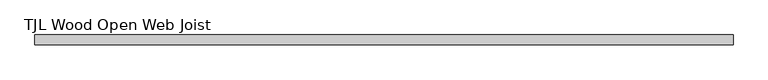
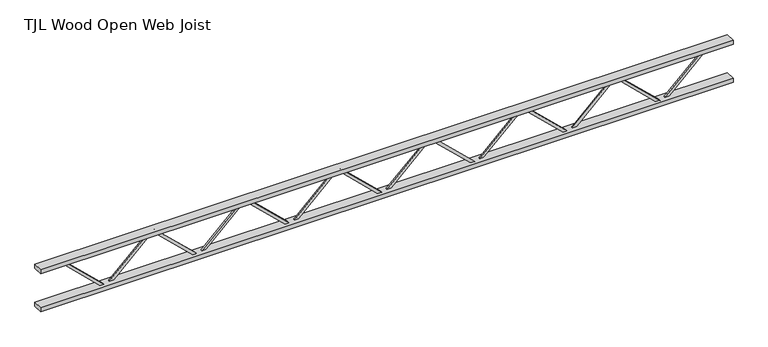
"""IFC4 building model written with IfcOpenShell, lengths in millimetres: beam geometry, TJL Wood Open Web Joist."""

from ifc_helpers import new_model, si_unit, frame, origin, place, context, project, spatial, polyline, outline, extrude, source, transform, mapped, element, save


def tjl_wood_open_web_joist_c41eeaf0(model_context):
    return source(origin(), model_context, "Body", "SweptSolid", [
        extrude(outline(polyline([(171.45, 2122.1473214), (196.85, 2122.1473214), (196.85, 2104.3636517), (-171.45, 1718.0341875), (-171.45, 1672.3178571), (-196.85, 1672.3178571), (-196.85, 1728.2015268), (171.45, 2114.5309911), (171.45, 2122.1473214)])), frame((0.0, 0.0, 0.0), z_axis=(0.0, 1.0, 0.0), x_axis=(0.0, 0.0, 1.0)), (0.0, 0.0, 1.0), 12.7),
        extrude(outline(polyline([(196.85, 1273.2883929), (171.45, 1273.2883929), (171.45, 1280.9047232), (-196.85, 1667.2341875), (-196.85, 1723.1178571), (-171.45, 1723.1178571), (-171.45, 1677.4015268), (196.85, 1291.0720625), (196.85, 1273.2883929)])), frame((0.0, -12.7, 0.0), z_axis=(0.0, 1.0, 0.0), x_axis=(0.0, 0.0, 1.0)), (0.0, 0.0, 1.0), 12.7),
        extrude(outline(polyline([(171.45, 1273.2883929), (196.85, 1273.2883929), (196.85, 1255.5047232), (-171.45, 869.1752589), (-171.45, 823.4589286), (-196.85, 823.4589286), (-196.85, 879.3425983), (171.45, 1265.6720625), (171.45, 1273.2883929)])), frame((0.0, 0.0, 0.0), z_axis=(0.0, 1.0, 0.0), x_axis=(0.0, 0.0, 1.0)), (0.0, 0.0, 1.0), 12.7),
        extrude(outline(polyline([(196.85, 424.4294643), (171.45, 424.4294643), (171.45, 432.0457946), (-196.85, 818.3752589), (-196.85, 874.2589286), (-171.45, 874.2589286), (-171.45, 828.5425983), (196.85, 442.213134), (196.85, 424.4294643)])), frame((0.0, -12.7, 0.0), z_axis=(0.0, 1.0, 0.0), x_axis=(0.0, 0.0, 1.0)), (0.0, 0.0, 1.0), 12.7),
        extrude(outline(polyline([(171.45, 424.4294643), (196.85, 424.4294643), (196.85, 406.6457946), (-171.45, 20.3163303), (-171.45, -25.4), (-196.85, -25.4), (-196.85, 30.4836697), (171.45, 416.813134), (171.45, 424.4294643)])), frame((0.0, 0.0, 0.0), z_axis=(0.0, 1.0, 0.0), x_axis=(0.0, 0.0, 1.0)), (0.0, 0.0, 1.0), 12.7),
        extrude(outline(polyline([(196.85, -424.4294643), (171.45, -424.4294643), (171.45, -416.813134), (-196.85, -30.4836697), (-196.85, 25.4), (-171.45, 25.4), (-171.45, -20.3163303), (196.85, -406.6457946), (196.85, -424.4294643)])), frame((0.0, -12.7, 0.0), z_axis=(0.0, 1.0, 0.0), x_axis=(0.0, 0.0, 1.0)), (0.0, 0.0, 1.0), 12.7),
        extrude(outline(polyline([(171.45, -424.4294643), (196.85, -424.4294643), (196.85, -442.213134), (-171.45, -828.5425983), (-171.45, -874.2589286), (-196.85, -874.2589286), (-196.85, -818.3752589), (171.45, -432.0457946), (171.45, -424.4294643)])), frame((0.0, 0.0, 0.0), z_axis=(0.0, 1.0, 0.0), x_axis=(0.0, 0.0, 1.0)), (0.0, 0.0, 1.0), 12.7),
        extrude(outline(polyline([(196.85, -1273.2883929), (171.45, -1273.2883929), (171.45, -1265.6720625), (-196.85, -879.3425983), (-196.85, -823.4589286), (-171.45, -823.4589286), (-171.45, -869.1752589), (196.85, -1255.5047232), (196.85, -1273.2883929)])), frame((0.0, -12.7, 0.0), z_axis=(0.0, 1.0, 0.0), x_axis=(0.0, 0.0, 1.0)), (0.0, 0.0, 1.0), 12.7),
        extrude(outline(polyline([(171.45, -1273.2883929), (196.85, -1273.2883929), (196.85, -1291.0720625), (-171.45, -1677.4015268), (-171.45, -1723.1178571), (-196.85, -1723.1178571), (-196.85, -1667.2341875), (171.45, -1280.9047232), (171.45, -1273.2883929)])), frame((0.0, 0.0, 0.0), z_axis=(0.0, 1.0, 0.0), x_axis=(0.0, 0.0, 1.0)), (0.0, 0.0, 1.0), 12.7),
        extrude(outline(polyline([(196.85, -2122.1473214), (171.45, -2122.1473214), (171.45, -2114.5309911), (-196.85, -1728.2015268), (-196.85, -1672.3178571), (-171.45, -1672.3178571), (-171.45, -1718.0341875), (196.85, -2104.3636517), (196.85, -2122.1473214)])), frame((0.0, -12.7, 0.0), z_axis=(0.0, 1.0, 0.0), x_axis=(0.0, 0.0, 1.0)), (0.0, 0.0, 1.0), 12.7),
        extrude(outline(polyline([(171.45, 2971.00625), (196.85, 2971.00625), (196.85, 2953.2225803), (-171.45, 2566.893116), (-171.45, 2521.1767857), (-196.85, 2521.1767857), (-196.85, 2577.0604554), (171.45, 2963.3899197), (171.45, 2971.00625)])), frame((0.0, 0.0, 0.0), z_axis=(0.0, 1.0, 0.0), x_axis=(0.0, 0.0, 1.0)), (0.0, 0.0, 1.0), 12.7),
        extrude(outline(polyline([(196.85, 2122.1473214), (171.45, 2122.1473214), (171.45, 2129.7636517), (-196.85, 2516.093116), (-196.85, 2571.9767857), (-171.45, 2571.9767857), (-171.45, 2526.2604554), (196.85, 2139.9309911), (196.85, 2122.1473214)])), frame((0.0, -12.7, 0.0), z_axis=(0.0, 1.0, 0.0), x_axis=(0.0, 0.0, 1.0)), (0.0, 0.0, 1.0), 12.7),
        extrude(outline(polyline([(171.45, -2122.1473214), (196.85, -2122.1473214), (196.85, -2139.9309911), (-171.45, -2526.2604554), (-171.45, -2571.9767857), (-196.85, -2571.9767857), (-196.85, -2516.093116), (171.45, -2129.7636517), (171.45, -2122.1473214)])), frame((0.0, 0.0, 0.0), z_axis=(0.0, 1.0, 0.0), x_axis=(0.0, 0.0, 1.0)), (0.0, 0.0, 1.0), 12.7),
        extrude(outline(polyline([(196.85, -2971.00625), (171.45, -2971.00625), (171.45, -2963.3899197), (-196.85, -2577.0604554), (-196.85, -2521.1767857), (-171.45, -2521.1767857), (-171.45, -2566.893116), (196.85, -2953.2225803), (196.85, -2971.00625)])), frame((0.0, -12.7, 0.0), z_axis=(0.0, 1.0, 0.0), x_axis=(0.0, 0.0, 1.0)), (0.0, 0.0, 1.0), 12.7),
        extrude(outline(polyline([(3174.20625, 44.45), (3174.20625, -44.45), (-3174.20625, -44.45), (-3174.20625, 44.45), (3174.20625, 44.45)])), frame((0.0, 0.0, 165.1), z_axis=(0.0, 0.0, 1.0), x_axis=(1.0, 0.0, 0.0)), (0.0, 0.0, 1.0), 38.1),
        extrude(outline(polyline([(3174.20625, 44.45), (3174.20625, -44.45), (-3174.20625, -44.45), (-3174.20625, 44.45), (3174.20625, 44.45)])), frame((0.0, 0.0, -203.2), z_axis=(0.0, 0.0, 1.0), x_axis=(1.0, 0.0, 0.0)), (0.0, 0.0, 1.0), 38.1),
    ])


if __name__ == "__main__":
    model = new_model("IFC4")
    model_context = context("Model", 3, world=origin())
    ifc_project = project(units=[si_unit("LENGTHUNIT", "METRE", prefix="MILLI")], contexts=[model_context])
    site = spatial("IfcSite", under=ifc_project)
    building = spatial("IfcBuilding", under=site)
    placement = place(None, origin())
    tjl_wood_open_web_joist_shape = tjl_wood_open_web_joist_c41eeaf0(model_context)
    element("IfcBeam", 1, ObjectType="TJL Wood Open Web Joist : 16\" PREENGINEERED FLOOR TRUSS", at=placement, inside=building, context=model_context, shape_type="MappedRepresentation", body=[
        mapped(tjl_wood_open_web_joist_shape, transform((0.0, 0.0, 0.0), x_axis=(1.0, 0.0, 0.0), y_axis=(0.0, 1.0, 0.0), z_axis=(0.0, 0.0, 1.0))),
    ])
    save(model, "model.ifc")

# Revit data of these elements
# Type "TJL Wood Open Web Joist : 16\" PREENGINEERED FLOOR TRUSS"
#   Web Thickness = 0' - 1"
#   Web Leg = 0' - 1"
#   Start Offset [instance default] = 0' - 0"
#   Top Chord Start Extension [instance default] = 0' - 0"
#   PanelArrayLength [instance default] = 22' - 8"
#   Depth = 1' - 4"
#   PanelWidth [instance default] = 2' - 6.22222"
#   Offset Length 2 [instance default] = 0' - 8"
#   Offset Length 1 [instance default] = 0' - 8"
#   End Panel [instance default] = 0' - 8"
#   End Offset [instance default] = 0' - 0"
#   Top Chord End Extension [instance default] = 0' - 0"
#   Chord Width = 0' - 3 1/2"
#   Chord Depth = 0' - 1 1/2"
#   Bottom Chord Start Extension [instance default] = 0' - 0"
#   Bottom Chord End Extension [instance default] = 0' - 0"
#   Length [instance default] = 24' - 0"
#   PanelArrayNum [instance default] = 9
#   Web Rendering Material = none
#   Structural Material = none
#   Assembly Code = ""
# Element 1 (IfcBeam, "TJL Wood Open Web Joist : 16\" PREENGINEERED FLOOR TRUSS")
#   PanelArrayLength = 19' - 5 15/16"
#   PanelWidth = 2' - 9.41964"
#   PanelArrayNum = 7
